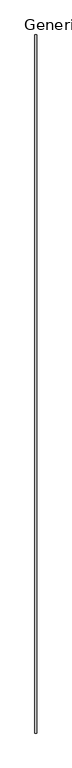
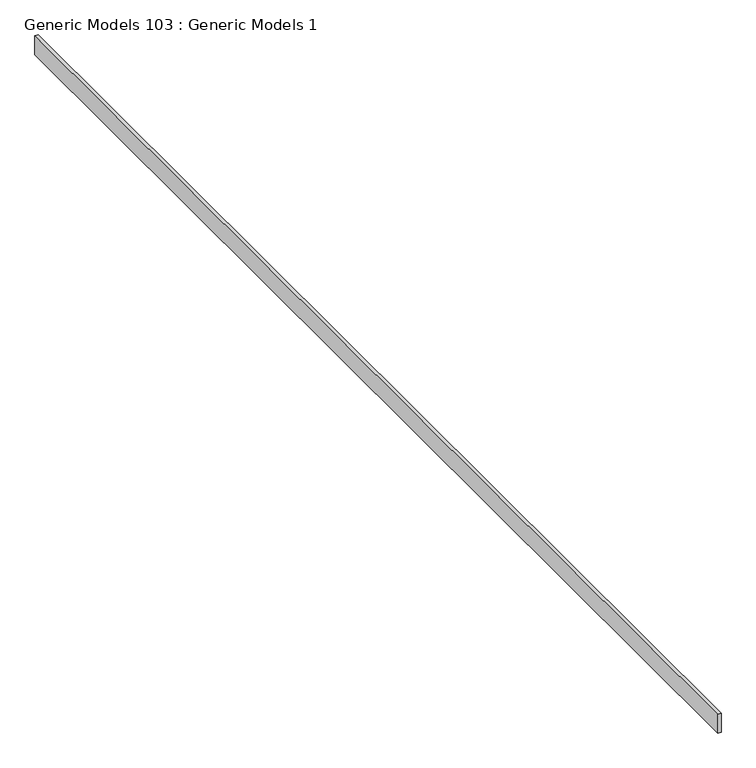
"""IFC4 building model written with IfcOpenShell, lengths in millimetres: proxy geometry, Generic Models 103 : Generic Models 1."""

from ifc_helpers import new_model, si_unit, frame, origin, place, context, project, spatial, polyline, outline, extrude, source, transform, mapped, element, save


def generic_models_103_generic_models_1_f31dc1f6(model_context):
    return source(origin(), model_context, "Body", "SweptSolid", [
        extrude(outline(polyline([(-5137.1966296, 7054.2769662), (-5099.0966296, 7054.2769662), (-5099.0966296, -7068.1230338), (-5137.1966296, -7068.1230338), (-5137.1966296, 7054.2769662)])), frame((0.0, 0.0, 126382.2085), z_axis=(0.0, 0.0, 1.0), x_axis=(1.0, 0.0, 0.0)), (0.0, 0.0, 1.0), 234.95),
    ])


if __name__ == "__main__":
    model = new_model("IFC4")
    model_context = context("Model", 3, world=origin())
    ifc_project = project(units=[si_unit("LENGTHUNIT", "METRE", prefix="MILLI")], contexts=[model_context])
    site = spatial("IfcSite", under=ifc_project)
    building = spatial("IfcBuilding", under=site)
    placement = place(None, origin())
    generic_models_103_generic_models_1_shape = generic_models_103_generic_models_1_f31dc1f6(model_context)
    element("IfcBuildingElementProxy", 1, Name="Generic Models 103 : Generic Models 1", ObjectType="Generic Models 103 : Generic Models 1", at=placement, inside=building, context=model_context, shape_type="MappedRepresentation", body=[
        mapped(generic_models_103_generic_models_1_shape, transform((0.0, 0.0, 0.0), x_axis=(1.0, 0.0, 0.0), y_axis=(0.0, 1.0, 0.0), z_axis=(0.0, 0.0, 1.0))),
    ])
    save(model, "model.ifc")

# Revit data of these elements
# Element 1 (IfcBuildingElementProxy, "Generic Models 103 : Generic Models 1")
#   Materials on its faces: "_2X STRUCTURAL BLOCKING (SEE STRUCT. DWGS)"
# Materials
#   "_2X STRUCTURAL BLOCKING (SEE STRUCT. DWGS)": class "Generic", colour RGB 177 130 114, transparency 0, Cost = 0
